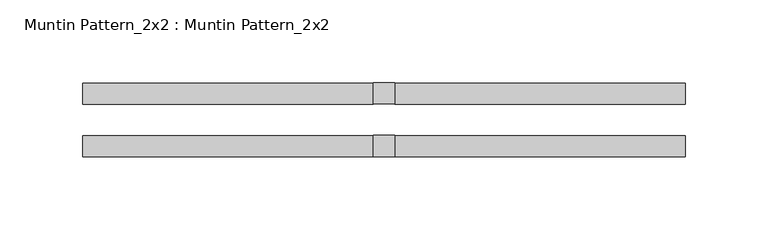
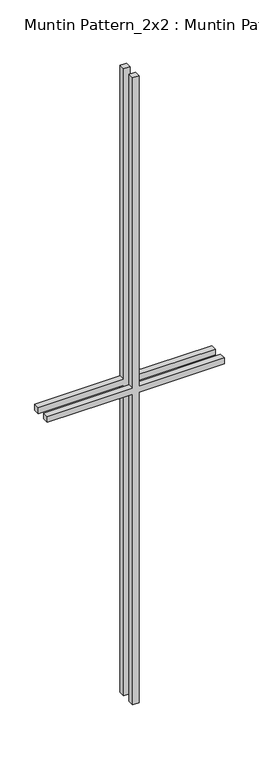
"""IFC4 building model written with IfcOpenShell, lengths in millimetres: proxy geometry, Muntin Pattern_2x2 : Muntin Pattern_2x2."""

from ifc_helpers import new_model, si_unit, frame, origin, place, context, project, spatial, polyline, outline, extrude, source, transform, mapped, element, save


def muntin_pattern_2x2_muntin_pattern_2x2_cbe63feb(model_context):
    return source(origin(), model_context, "Body", "SweptSolid", [
        extrude(outline(polyline([(686.5, -6.35), (686.5, -181.7375), (673.8, -181.7375), (673.8, -6.35), (0.0, -6.35), (0.0, 6.35), (673.8, 6.35), (673.8, 181.7375), (686.5, 181.7375), (686.5, 6.35), (1360.3, 6.35), (1360.3, -6.35), (686.5, -6.35)])), frame((0.0, -22.225, 0.0), z_axis=(0.0, 1.0, 0.0), x_axis=(0.0, 0.0, 1.0)), (0.0, 0.0, 1.0), 12.7),
        extrude(outline(polyline([(686.5, -6.35), (686.5, -181.7375), (673.8, -181.7375), (673.8, -6.35), (0.0, -6.35), (0.0, 6.35), (673.8, 6.35), (673.8, 181.7375), (686.5, 181.7375), (686.5, 6.35), (1360.3, 6.35), (1360.3, -6.35), (686.5, -6.35)])), frame((0.0, 9.525, 0.0), z_axis=(0.0, 1.0, 0.0), x_axis=(0.0, 0.0, 1.0)), (0.0, 0.0, 1.0), 12.7),
    ])


if __name__ == "__main__":
    model = new_model("IFC4")
    model_context = context("Model", 3, world=origin())
    ifc_project = project(units=[si_unit("LENGTHUNIT", "METRE", prefix="MILLI")], contexts=[model_context])
    site = spatial("IfcSite", under=ifc_project)
    building = spatial("IfcBuilding", under=site)
    placement = place(None, origin())
    muntin_pattern_2x2_muntin_pattern_2x2_shape = muntin_pattern_2x2_muntin_pattern_2x2_cbe63feb(model_context)
    element("IfcBuildingElementProxy", 1, Name="Muntin Pattern_2x2 : Muntin Pattern_2x2", ObjectType="Muntin Pattern_2x2 : Muntin Pattern_2x2", at=placement, inside=building, context=model_context, shape_type="MappedRepresentation", body=[
        mapped(muntin_pattern_2x2_muntin_pattern_2x2_shape, transform((0.0, 0.0, 0.0), x_axis=(1.0, 0.0, 0.0), y_axis=(0.0, 1.0, 0.0), z_axis=(0.0, 0.0, 1.0))),
    ])
    save(model, "model.ifc")

# Revit data of these elements
# Type "Muntin Pattern_2x2 : Muntin Pattern_2x2"
#   Width [instance default] = 1.2192 m
#   Thickness = 0.0127 m
#   Height [instance default] = 1.2192 m
#   Distance = 0.01905 m
#   Interior Material [instance default] = none
#   Exterior Material [instance default] = none
# Element 1 (IfcBuildingElementProxy, "Muntin Pattern_2x2 : Muntin Pattern_2x2")
#   Width = 0.363475 m
#   Height = 1.3603 m
#   Interior Material = Wood - Stained
#   Exterior Material = Clad - White
#   Materials on its faces: "Clad - White", "Wood - Stained"
# Materials
#   "Clad - White": class "Wood", colour RGB 242 242 238, transparency 0, Cost = 0
#   "Wood - Stained": class "Wood", colour RGB 224 178 126, transparency 0, Cost = 0
